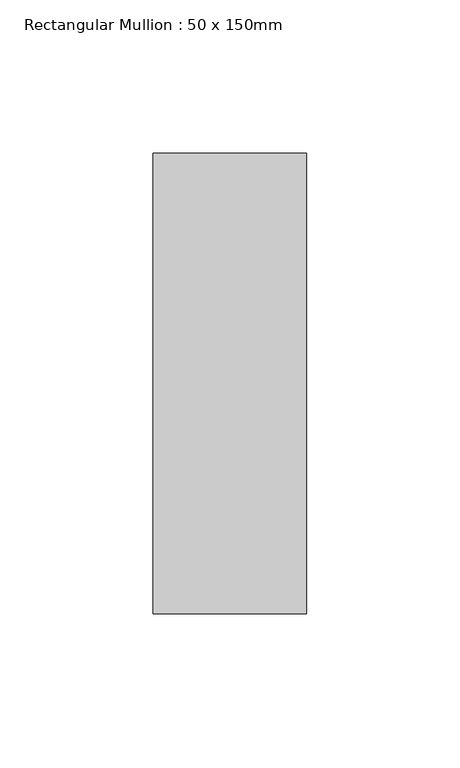
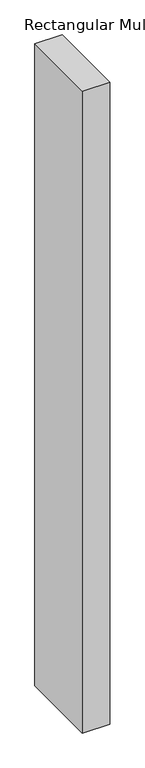
"""IFC4 building model written with IfcOpenShell, lengths in millimetres: member geometry, Rectangular Mullion : 50 x 150mm."""

import ifcopenshell
import ifcopenshell.guid

model = None  # the IFC model being written
_history = None  # IfcOwnerHistory: only IFC2X3 demands one
_inside = {}  # id of a spatial element -> (the spatial element, [elements in it])
_under = {}  # id of a project, library or spatial element -> (it, [spatial elements below it])
_declared = {}  # id of a project -> (the project, [libraries it declares])
_typed = {}  # id of a type object -> (the type object, [elements of that type])
_made_of = {}  # id of a material, layer set ... -> (it, [elements and type objects made of it])


def new_model(schema):
    """Start an empty IFC model of exactly this schema.

    Asked for "IFC4X3", IfcOpenShell would pick the latest addendum, in which some entities
    have other attributes; the version numbers below select the first issue.
    IFC2X3 requires an IfcOwnerHistory on every rooted entity: one is made here for all.
    """
    global model, _history
    if schema == "IFC4X3":
        model = ifcopenshell.file(schema_version=(4, 3, 0, 0))
    else:
        model = ifcopenshell.file(schema=schema)
    _inside.clear()
    _under.clear()
    _declared.clear()
    _typed.clear()
    _made_of.clear()
    _history = None
    if model.schema == "IFC2X3":
        org = make("IfcOrganization", Name="unknown")
        user = make(
            "IfcPersonAndOrganization",
            ThePerson=make("IfcPerson", FamilyName="unknown"),
            TheOrganization=org,
        )
        app = make(
            "IfcApplication",
            ApplicationDeveloper=org,
            Version="unknown",
            ApplicationFullName="unknown",
            ApplicationIdentifier="unknown",
        )
        _history = make(
            "IfcOwnerHistory",
            OwningUser=user,
            OwningApplication=app,
            ChangeAction="ADDED",
            CreationDate=0,
        )
    return model


def make(cls, **values):
    """One entity of the class cls with the attributes given. An attribute that is None is left unset."""
    return model.create_entity(
        cls, **{name: value for name, value in values.items() if value is not None}
    )


def rooted(cls, **values):
    """An entity with a GlobalId (a new one), such as an element, a storey or a relation."""
    return make(cls, GlobalId=ifcopenshell.guid.new(), OwnerHistory=_history, **values)


def si_unit(unit_type, name, prefix=None):
    """IfcSIUnit, for example si_unit("LENGTHUNIT", "METRE", prefix="MILLI")."""
    return make("IfcSIUnit", UnitType=unit_type, Prefix=prefix, Name=name)


def assignment(units):
    """IfcUnitAssignment: the units of a project."""
    return None if units is None else make("IfcUnitAssignment", Units=units)


def point(xyz):
    """IfcCartesianPoint."""
    return None if xyz is None else make("IfcCartesianPoint", Coordinates=xyz)


def direction(xyz):
    """IfcDirection."""
    return None if xyz is None else make("IfcDirection", DirectionRatios=xyz)


def frame(location, z_axis=None, x_axis=None):
    """IfcAxis2Placement3D, a coordinate frame: its origin and axes. An axis left out is left unset."""
    return make(
        "IfcAxis2Placement3D",
        Location=point(location),
        Axis=direction(z_axis),
        RefDirection=direction(x_axis),
    )


def origin():
    """The frame at (0, 0, 0) with its axes left unset."""
    return frame((0.0, 0.0, 0.0))


def place(relative_to, where):
    """IfcLocalPlacement: puts the frame where relative to a parent placement (None: the world)."""
    return make(
        "IfcLocalPlacement", PlacementRelTo=relative_to, RelativePlacement=where
    )


def context(
    kind, dimensions, precision=None, world=None, true_north=None, identifier=None
):
    """IfcGeometricRepresentationContext, for example the 3D "Model" context."""
    return make(
        "IfcGeometricRepresentationContext",
        ContextIdentifier=identifier,
        ContextType=kind,
        CoordinateSpaceDimension=dimensions,
        Precision=precision,
        WorldCoordinateSystem=world,
        TrueNorth=true_north,
    )


def project(units=None, contexts=None):
    """IfcProject with its units and contexts."""
    return rooted(
        "IfcProject",
        Name="project",
        RepresentationContexts=contexts,
        UnitsInContext=assignment(units),
    )


def spatial(cls, under=None, at=None, **own):
    """A site, building, storey or space (cls), placed at a placement, below another one or the project."""
    s = rooted(cls, ObjectPlacement=at, **own)
    if under is not None:
        _under.setdefault(under.id(), (under, []))[1].append(s)
    return s


def polyline(points):
    """IfcPolyline through the points."""
    return make("IfcPolyline", Points=[point(p) for p in points])


def outline(outer, holes=None, kind="AREA"):
    """IfcArbitraryClosedProfileDef: a profile drawn as a closed curve; with holes, ...WithVoids."""
    if holes is None:
        return make("IfcArbitraryClosedProfileDef", ProfileType=kind, OuterCurve=outer)
    return make(
        "IfcArbitraryProfileDefWithVoids",
        ProfileType=kind,
        OuterCurve=outer,
        InnerCurves=holes,
    )


def extrude(swept, where, along, depth):
    """IfcExtrudedAreaSolid: the profile swept, set in the frame where, extruded along a direction by depth."""
    return make(
        "IfcExtrudedAreaSolid",
        SweptArea=swept,
        Position=where,
        ExtrudedDirection=direction(along),
        Depth=depth,
    )


def shape(context_of_items, identifier, shape_type, items):
    """IfcShapeRepresentation: the items that make up one representation, for example the "Body"."""
    return make(
        "IfcShapeRepresentation",
        ContextOfItems=context_of_items,
        RepresentationIdentifier=identifier,
        RepresentationType=shape_type,
        Items=items,
    )


def source(mapping_origin, context_of_items, identifier, shape_type, items):
    """IfcRepresentationMap: a shape defined once, which mapped items show again and again."""
    return make(
        "IfcRepresentationMap",
        MappingOrigin=mapping_origin,
        MappedRepresentation=shape(context_of_items, identifier, shape_type, items),
    )


def transform(
    local_origin,
    x_axis=None,
    y_axis=None,
    z_axis=None,
    scale=None,
    scale2=None,
    scale3=None,
    uniform=True,
):
    """IfcCartesianTransformationOperator3D, or its non-uniform kind. x_axis, y_axis, z_axis: its Axis1, 2, 3."""
    if uniform:
        return make(
            "IfcCartesianTransformationOperator3D",
            Axis1=direction(x_axis),
            Axis2=direction(y_axis),
            LocalOrigin=point(local_origin),
            Scale=scale,
            Axis3=direction(z_axis),
        )
    return make(
        "IfcCartesianTransformationOperator3DnonUniform",
        Axis1=direction(x_axis),
        Axis2=direction(y_axis),
        LocalOrigin=point(local_origin),
        Scale=scale,
        Axis3=direction(z_axis),
        Scale2=scale2,
        Scale3=scale3,
    )


def mapped(mapping_source, mapping_target):
    """IfcMappedItem: shows the shape of a source again, moved by a transform."""
    return make(
        "IfcMappedItem", MappingSource=mapping_source, MappingTarget=mapping_target
    )


def made_of(thing, what):
    """Note that an element or type object is made of a material, layer set ...; save() writes the relation."""
    if what is not None:
        _made_of.setdefault(what.id(), (what, []))[1].append(thing)
    return thing


def element(
    cls,
    number,
    at=None,
    inside=None,
    cuts=None,
    type_object=None,
    material=None,
    context=None,
    identifier="Body",
    shape_type=None,
    held_by="IfcProductDefinitionShape",
    body=None,
    shapes=None,
    **own,
):
    """One element of the class cls, such as IfcWall. Its Tag is "e" and its number.

    at: its placement. inside: the storey or other place that contains it. cuts: it is an
    opening in that element (IfcRelVoidsElement). A single representation is given by context,
    identifier, shape_type and body (its items); several are given by shapes. held_by: the class
    of the entity that holds the representations. save() writes the other relations.
    """
    e = rooted(cls, Tag="e%d" % number, ObjectPlacement=at, **own)
    if body is not None:
        shapes = [shape(context, identifier, shape_type, body)]
    if shapes is not None:
        e.Representation = make(held_by, Representations=shapes)
    if inside is not None:
        _inside.setdefault(inside.id(), (inside, []))[1].append(e)
    if cuts is not None:
        rooted(
            "IfcRelVoidsElement", RelatingBuildingElement=cuts, RelatedOpeningElement=e
        )
    if type_object is not None:
        _typed.setdefault(type_object.id(), (type_object, []))[1].append(e)
    return made_of(e, material)


def aggregate(whole, parts):
    """IfcRelAggregates: a whole, such as a stair, and the parts it consists of."""
    return rooted("IfcRelAggregates", RelatingObject=whole, RelatedObjects=parts)


def save(model, path):
    """Write the relations noted so far, then the file.

    IfcRelAggregates (storeys below a building ...), IfcRelContainedInSpatialStructure (elements
    in a storey), IfcRelDefinesByType, IfcRelAssociatesMaterial and IfcRelDeclares: one each for
    every whole, place, type object, material and project.
    """
    for whole, parts in _under.values():
        aggregate(whole, parts)
    for where, things in _inside.values():
        rooted(
            "IfcRelContainedInSpatialStructure",
            RelatedElements=things,
            RelatingStructure=where,
        )
    for kind, things in _typed.values():
        rooted("IfcRelDefinesByType", RelatedObjects=things, RelatingType=kind)
    for what, things in _made_of.values():
        rooted("IfcRelAssociatesMaterial", RelatedObjects=things, RelatingMaterial=what)
    for by, libraries in _declared.values():
        rooted("IfcRelDeclares", RelatingContext=by, RelatedDefinitions=libraries)
    model.write(path)


def rectangular_mullion_50_x_150mm_23e890aa(model_context):
    return source(origin(), model_context, "Body", "SweptSolid", [
        extrude(outline(polyline([(25.0, 75.0), (25.0, -75.0), (-25.0, -75.0), (-25.0, 75.0), (25.0, 75.0)])), frame((0.0, 0.0, -1240.0000002), z_axis=(0.0, 0.0, 1.0), x_axis=(1.0, 0.0, 0.0)), (0.0, 0.0, 1.0), 1240.0000002),
    ])


if __name__ == "__main__":
    model = new_model("IFC4")
    model_context = context("Model", 3, world=origin())
    ifc_project = project(units=[si_unit("LENGTHUNIT", "METRE", prefix="MILLI")], contexts=[model_context])
    site = spatial("IfcSite", under=ifc_project)
    building = spatial("IfcBuilding", under=site)
    placement = place(None, origin())
    rectangular_mullion_50_x_150mm_shape = rectangular_mullion_50_x_150mm_23e890aa(model_context)
    element("IfcMember", 1, ObjectType="Rectangular Mullion : 50 x 150mm", at=placement, inside=building, context=model_context, shape_type="MappedRepresentation", body=[
        mapped(rectangular_mullion_50_x_150mm_shape, transform((0.0, 0.0, 0.0), x_axis=(1.0, 0.0, 0.0), y_axis=(0.0, 1.0, 0.0), z_axis=(0.0, 0.0, 1.0))),
    ])
    save(model, "model.ifc")

# Revit data of these elements
# Type "Rectangular Mullion : 50 x 150mm"
#   built-in parameter 1007304 = 0.492126 (stored number, unit not read)
#   built-in parameter 1007301 = 0.082021 (stored number, unit not read)
#   built-in parameter 1007300 = 0.082021 (stored number, unit not read)
# Element 1 (IfcMember, "Rectangular Mullion : 50 x 150mm")
#   Materials on its faces: "Aluminium"
# Materials
#   "Aluminium": class "Metal", colour RGB 247 247 247, transparency 0, Description = "Aluminium 6061", Cost = 0
